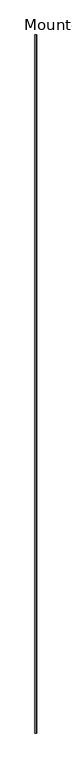
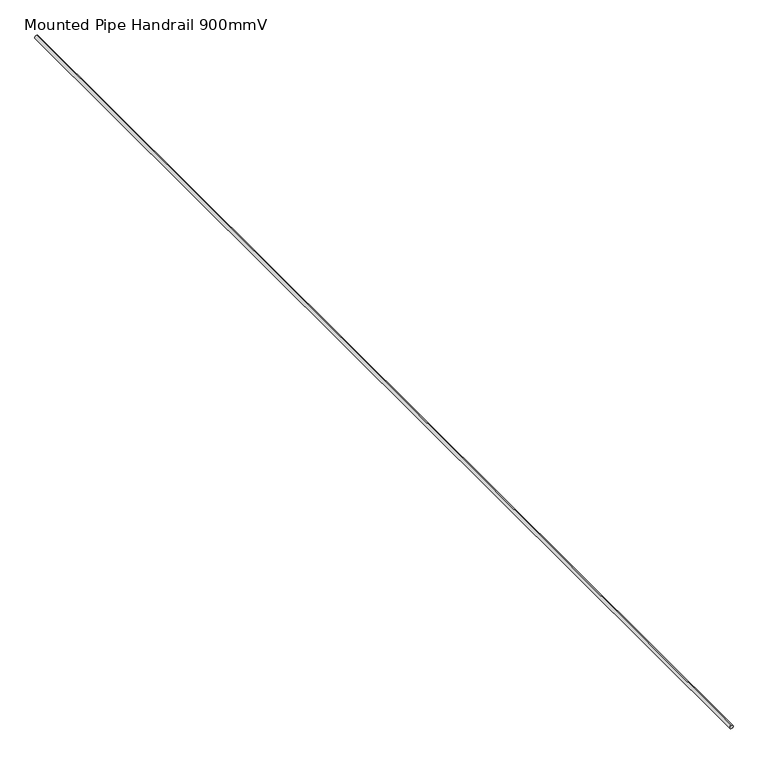
"""IFC4 building model written with IfcOpenShell, lengths in millimetres: railing geometry, Mounted Pipe Handrail 900mmV."""

from ifc_helpers import new_model, si_unit, point, frame, origin, place, context, project, spatial, ellipse_curve, trimmed, source, transform, mapped, element, save
from ifc_brep_helpers import plane_surface, extruded_surface, advanced_brep


def mounted_pipe_handrail_900mmv_ce20a273(model_context):
    return source(origin(), model_context, "Body", "AdvancedBrep", [
        advanced_brep(
        [(-13673.1278716, 5753.2922384, 1919.6965624), (-13673.1278716, 5753.2922384, 1881.5965624), (-13673.1278716, 18753.2922384, 1919.6965624), (-13673.1278716, 18753.2922384, 1881.5965624)],
        [
            (0, 1, ellipse_curve(frame((-13673.1278716, 5753.2922384, 1900.6465624), z_axis=(0.0, -1.0, 0.0), x_axis=(0.0, 0.0, -1.0)), 19.05, 19.05)),
            (1, 0, ellipse_curve(frame((-13673.1278716, 5753.2922384, 1900.6465624), z_axis=(0.0, -1.0, 0.0), x_axis=(0.0, 0.0, -1.0)), 19.05, 19.05)),
            (2, 3, ellipse_curve(frame((-13673.1278716, 18753.2922384, 1900.6465624), z_axis=(0.0, 1.0, 0.0), x_axis=(0.0, 0.0, -1.0)), 19.05, 19.05)),
            (3, 2, ellipse_curve(frame((-13673.1278716, 18753.2922384, 1900.6465624), z_axis=(0.0, 1.0, 0.0), x_axis=(0.0, 0.0, -1.0)), 19.05, 19.05)),
            (0, 2),
            (3, 1),
        ],
        [
            plane_surface(frame((-13673.1278716, 5753.2922384, 1900.6465624), z_axis=(0.0, -1.0, 0.0), x_axis=(0.0, 0.0, 1.0))),
            plane_surface(frame((-13673.1278716, 18753.2922384, 1900.6465624), z_axis=(0.0, 1.0, 0.0), x_axis=(0.0, 0.0, 1.0))),
            extruded_surface(trimmed(ellipse_curve(frame((-13673.1278716, 18753.2922384, 1900.6465624), z_axis=(0.0, -1.0, 0.0), x_axis=(0.0, 0.0, -1.0)), 19.05, 19.05), [point((-13673.1278716, 18753.2922384, 1919.6965624))], [point((-13673.1278716, 18753.2922384, 1881.5965624))], True, "CARTESIAN"), (0.0, -13000.0, 0.0), 13000.0),
            extruded_surface(trimmed(ellipse_curve(frame((-13673.1278716, 18753.2922384, 1900.6465624), z_axis=(0.0, -1.0, 0.0), x_axis=(0.0, 0.0, -1.0)), 19.05, 19.05), [point((-13673.1278716, 18753.2922384, 1881.5965624))], [point((-13673.1278716, 18753.2922384, 1919.6965624))], True, "CARTESIAN"), (0.0, -13000.0, 0.0), 13000.0),
        ],
        [
            (0, [[1, 2]]),
            (1, [[3, 4]]),
            (2, [[-1, 5, -4, 6]]),
            (3, [[-2, -6, -3, -5]]),
        ],
    ),
    ])


if __name__ == "__main__":
    model = new_model("IFC4")
    model_context = context("Model", 3, world=origin())
    ifc_project = project(units=[si_unit("LENGTHUNIT", "METRE", prefix="MILLI")], contexts=[model_context])
    site = spatial("IfcSite", under=ifc_project)
    building = spatial("IfcBuilding", under=site)
    placement = place(None, origin())
    mounted_pipe_handrail_900mmv_shape = mounted_pipe_handrail_900mmv_ce20a273(model_context)
    element("IfcRailing", 1, ObjectType="Mounted Pipe Handrail 900mmV", at=placement, inside=building, context=model_context, shape_type="MappedRepresentation", body=[
        mapped(mounted_pipe_handrail_900mmv_shape, transform((0.0, 0.0, 0.0), x_axis=(1.0, 0.0, 0.0), y_axis=(0.0, 1.0, 0.0), z_axis=(0.0, 0.0, 1.0))),
    ])
    save(model, "model.ifc")

# Revit data of these elements
# Element 1 (IfcRailing, "Mounted Pipe Handrail 900mmV")
#   Materials on its faces: "1 1/2\" DIA. HANDRAIL (1 1/2\" MIN. CLEAR FROM WALL)"
# Materials
#   "1 1/2\" DIA. HANDRAIL (1 1/2\" MIN. CLEAR FROM WALL)": class "Unassigned", colour RGB 199 199 199, transparency 0, Cost = 0
